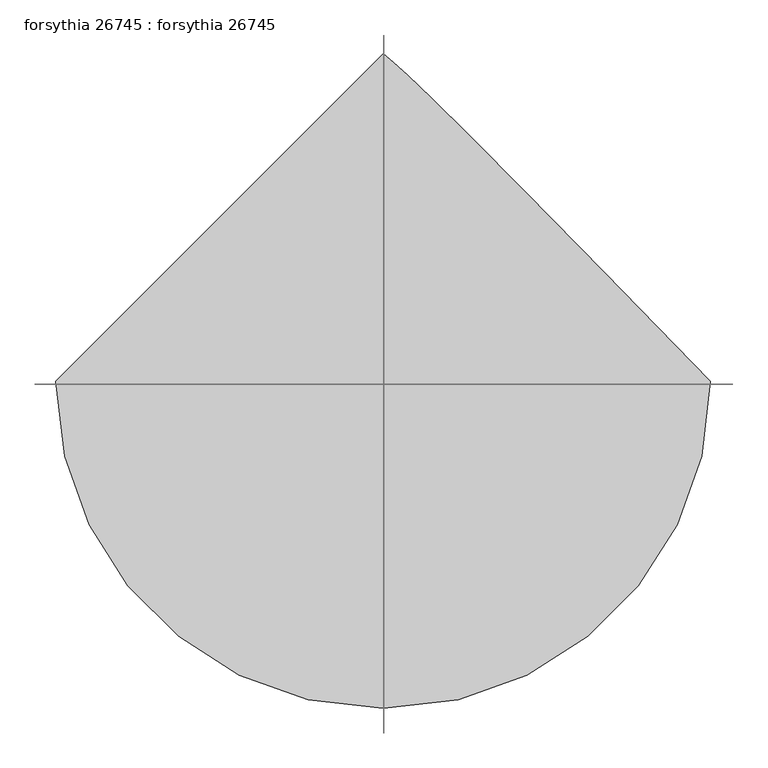
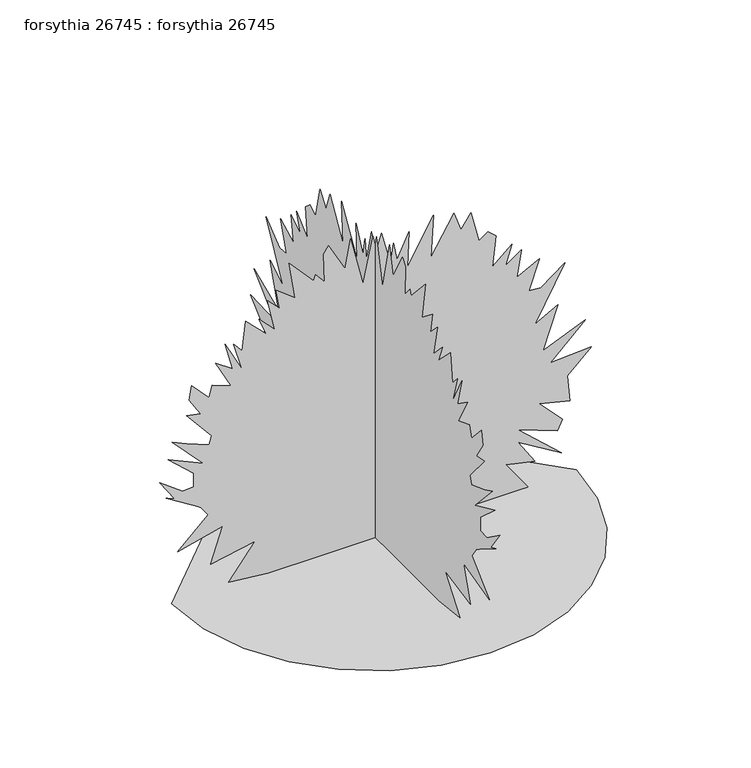
"""IFC4 building model written with IfcOpenShell, lengths in millimetres: proxy geometry, forsythia 26745 : forsythia 26745."""

from ifc_helpers import new_model, si_unit, origin, place, context, project, spatial, triangles, source, transform, mapped, element, save


def forsythia_26745_forsythia_26745_3ae10d36(model_context):
    return source(origin(), model_context, "Body", "Tessellation", [
        triangles([(-1519.5040535, 0.0, 0.0002833), (-1479.3336857, -348.1690825, 0.0002833), (-1364.9291862, -667.9078508, 0.0002833), (-1185.447191, -950.0545097, 0.0002833), (-950.0545097, -1185.447191, 0.0002833), (-667.9078508, -1364.9291862, 0.0002833), (-348.1690825, -1479.3336857, 0.0002833), (6.64e-05, -1519.5040535, 0.0002833), (348.1690825, -1479.3336857, 0.0002833), (667.9078508, -1364.9291862, 0.0002833), (950.0545097, -1185.447191, 0.0002833), (1185.447191, -950.0545097, 0.0002833), (1364.9291862, -667.9078508, 0.0002833), (1479.3336857, -348.1690825, 0.0002833), (1519.5040535, 0.0001328, 0.0002833), (1025.698439, 506.5233338, 0.0002833), (659.6172232, 879.4549673, 0.0002833), (399.9699903, 1141.05804, 0.0002833), (225.4722113, 1313.5981625, 0.0002833), (114.8360501, 1419.3438881, 0.0002833), (46.774248, 1480.5555588, 0.0002833), (-0.0001993, 1519.5040535, 0.0002833), (-792.3428427, -13.4822871, 0.037948), (-1099.2418425, -13.4822621, 31.9687972), (-901.0348274, -13.4822871, 287.7194292), (-1233.5117718, -13.4822871, 223.7813261), (-1143.9993576, -13.4822871, 492.3196223), (-1482.8669003, -13.4822871, 409.2003862), (-1252.691415, -13.482312, 620.1937574), (-1310.2352863, -13.482312, 703.3130299), (-1565.9861, -13.482312, 863.1557442), (-1502.0490143, -13.482312, 837.5804157), (-1617.1342861, -13.482312, 1003.8188152), (-1444.505143, -13.482312, 875.9446438), (-1361.3859432, -13.482312, 882.3378582), (-1361.3859432, -13.482312, 991.0299156), (-1553.1972004, -13.4823382, 1163.6615295), (-1291.0531723, -13.4823382, 1042.1805725), (-1521.2286575, -13.4823382, 1291.5383171), (-1412.5366001, -13.4823382, 1240.3875149), (-1246.2982006, -13.4823382, 1176.4505018), (-1227.1160866, -13.4823382, 1240.3875149), (-1412.5366001, -13.4823382, 1464.1673149), (-1310.2352863, -13.4823382, 1444.987817), (-1393.3544861, -13.4823631, 1579.2552029), (-1374.1723721, -13.4823631, 1687.9497311), (-1246.2982006, -13.4823631, 1547.28666), (-1220.7228722, -13.4823631, 1636.7990742), (-1080.0597284, -13.4823631, 1585.6482719), (-1195.147471, -13.4823631, 1803.0374737), (-1067.2732996, -13.4823631, 1713.5250595), (-1124.8171709, -13.4823881, 1930.9116451), (-996.9429995, -13.4823631, 1687.9497311), (-1060.8800852, -13.4823881, 1905.3363167), (-996.9429995, -13.4823631, 1835.0060165), (-971.367671, -13.4823881, 2058.7858166), (-817.9181711, -13.4823881, 1905.3363167), (-869.0663572, -13.4823881, 2039.6061733), (-753.9785419, -13.4823881, 1918.1252163), (-805.1292715, -13.4823881, 2161.0871304), (-715.6167847, -13.4823881, 2071.5747162), (-741.1921858, -13.4823881, 2225.0242161), (-600.5290421, -13.4823881, 2116.3296879), (-645.2865572, -13.4824142, 2404.0490444), (-459.8659347, -13.4823881, 2199.4488876), (-447.0795422, -13.4823881, 2244.2063301), (-379.2689283, -13.4823881, 2162.8804802), (-385.6646862, -13.4824142, 2386.6602802), (-347.290248, -13.4824142, 2438.4078484), (-223.176294, -13.4824142, 2213.9981449), (-182.9654127, -13.4823631, 2435.1743248), (-90.8322191, -13.4823631, 2047.6376598), (-12.3045871, -13.4824142, 2397.6559753), (13.2704245, -13.4823881, 2276.174873), (51.6330312, -13.4824142, 2397.6559753), (115.5706256, -13.4823881, 2135.5118019), (141.1454544, -13.4823881, 2288.9613018), (166.7205467, -13.4823881, 2148.2982307), (256.2334877, -13.4824142, 2340.1119587), (243.445551, -13.4823881, 2065.1815018), (441.6515305, -13.4824142, 2404.0490444), (422.4693801, -13.4823881, 2077.9679306), (595.1010303, -13.4824142, 2365.6874325), (646.2517599, -13.4823881, 2218.6310017), (722.9777452, -13.4824142, 2327.3230591), (780.5216166, -13.4823881, 2084.361145), (850.8519167, -13.4823881, 2129.1185875), (908.395788, -13.4823881, 2077.9679306), (882.8204596, -13.4823631, 1841.399231), (1029.876745, -13.4823881, 1969.2734024), (978.7260881, -13.4823631, 1815.8239025), (1100.2070452, -13.4823881, 1898.9431023), (1068.2385023, -13.4823631, 1694.3429455), (1234.4769745, -13.4823631, 1783.8553596), (1157.7509165, -13.4823631, 1553.6797291), (1247.2634033, -13.4823631, 1547.28666), (1426.2882317, -13.4823631, 1681.5565166), (1202.5084316, -13.4823382, 1272.3560577), (1375.1400455, -13.4823382, 1368.2616863), (1260.0523029, -13.4823382, 1042.1805725), (1579.7377316, -13.4823382, 1176.4505018), (1317.5961742, -13.482312, 927.0928299), (1624.495174, -13.482312, 946.2749439), (1445.4703457, -13.482312, 780.0364717), (1464.6524597, -13.4822871, 575.436315), (1234.4769745, -13.482312, 632.9801863), (1407.1085884, -13.4822871, 447.5621435), (1368.7443604, -13.4822871, 370.838629), (1074.6317167, -13.4822871, 479.5306864), (1400.7129032, -13.4822871, 185.418824), (1074.6317167, -13.4822871, 383.6250578), (1202.5084316, -13.4822871, 185.418824), (985.1193026, -13.4822871, 236.568736), (1151.4898161, -13.4822871, 0.0386752), (19.664159, -13.4822621, 0.0001234), (3.6800653, -809.5031324, 0.0378489), (3.68004, -1116.4046757, 31.9687972), (3.6800653, -918.1977333, 287.7194292), (3.6800653, -1250.6720615, 223.7813261), (3.6800653, -1161.1596474, 492.3196223), (3.6800653, -1500.0298061, 409.2003862), (3.6800653, -1269.8541756, 620.1937574), (3.6800653, -1327.3980469, 703.3130299), (3.6800908, -1583.1463898, 863.1557442), (3.6800908, -1519.209304, 837.5804157), (3.6800908, -1634.2970467, 1003.8188152), (3.6800908, -1461.6654327, 875.9446438), (3.6800908, -1378.5487038, 882.3378582), (3.6800908, -1378.5487038, 991.0299156), (3.6800908, -1570.3599609, 1163.6615295), (3.6800908, -1308.2159328, 1042.1805725), (3.6800908, -1538.3914181, 1291.5383171), (3.6800908, -1429.6968899, 1240.3875149), (3.6800908, -1263.4609612, 1176.4505018), (3.6800908, -1244.2788471, 1240.3875149), (3.6800908, -1429.6968899, 1464.1673149), (3.6800908, -1327.3980469, 1444.987817), (3.6800908, -1410.5172466, 1579.2552029), (3.6801161, -1391.3351326, 1687.9497311), (3.6800908, -1263.4609612, 1547.28666), (3.6800908, -1237.8856327, 1636.7990742), (3.6800908, -1097.2225616, 1585.6508881), (3.6801161, -1212.3103043, 1803.0374737), (3.6800908, -1084.4361328, 1713.5250595), (3.6801161, -1141.9800041, 1930.9116451), (3.6800908, -1014.1032892, 1687.9497311), (3.6801161, -1078.0403749, 1905.3363167), (3.6800908, -1014.1032892, 1835.0060165), (3.6801161, -988.5305042, 2058.7858166), (3.6800908, -835.0784609, 1905.3363167), (3.6801161, -886.2291904, 2039.6061733), (3.6800908, -771.1413752, 1918.1252163), (3.6801161, -822.2921047, 2161.0871304), (3.6801161, -732.7796179, 2071.5747162), (3.6801161, -758.355019, 2225.0242161), (3.6801161, -617.6918753, 2116.3296879), (3.6801161, -662.446847, 2404.0490444), (3.6801161, -477.0287679, 2199.4488876), (3.6801161, -464.2423754, 2244.2063301), (3.6801161, -396.4317616, 2162.8804802), (3.6801161, -402.824976, 2386.6602802), (3.6801161, -364.4530812, 2438.4078484), (3.6801161, -240.3386185, 2213.9981449), (3.6800653, -200.1277554, 2435.1743248), (3.6800653, -107.994798, 2047.640276), (3.6801161, -29.4668878, 2397.6559753), (3.6800908, -3.8919275, 2276.174873), (3.6801161, 34.4707044, 2397.6559753), (3.6800908, 98.408301, 2135.5118019), (3.6800908, 123.9831299, 2288.9613018), (3.6800908, 149.5579678, 2148.3008469), (3.6800908, 239.0706363, 2340.1119587), (3.6800908, 226.2832264, 2065.1815018), (3.6800908, 424.4886972, 2404.0490444), (3.6800908, 405.3090903, 2077.9679306), (3.6800908, 577.9381971, 2365.6874325), (3.6800908, 629.0889267, 2218.6310017), (3.6800908, 705.814912, 2327.3256752), (3.6800908, 763.3587833, 2084.361145), (3.6800908, 833.6890835, 2129.1185875), (3.6800908, 891.2329548, 2077.9679306), (3.6800653, 865.6576263, 1841.399231), (3.6800653, 1012.7139118, 1969.2734024), (3.6800653, 961.5632549, 1815.8239025), (3.6800653, 1083.044212, 1898.9431023), (3.6800653, 1051.0756691, 1694.3429455), (3.6800653, 1217.3141413, 1783.8553596), (3.6800653, 1140.5880833, 1553.6797291), (3.6800653, 1230.1004974, 1547.28666), (3.6800653, 1409.1253258, 1681.5565166), (3.6800653, 1185.3455984, 1272.3560577), (3.6800653, 1357.977285, 1368.2616863), (3.68004, 1242.8895424, 1042.1805725), (3.68004, 1562.5774418, 1176.4505018), (3.68004, 1300.4334137, 927.0928299), (3.68004, 1607.3324135, 946.2749439), (3.68004, 1428.3075851, 780.0364717), (3.68004, 1447.4896992, 575.436315), (3.68004, 1217.3141413, 632.9801863), (3.6800145, 1389.9458279, 447.5621435), (3.6800145, 1351.5840706, 370.838629), (3.68004, 1057.471427, 479.5306864), (3.6800145, 1383.5526134, 185.4185696), (3.68004, 1057.471427, 383.6250578), (3.6800145, 1185.3455984, 185.4185696), (3.6800145, 967.9590128, 236.568736), (3.68004, 1134.3269829, 0.038518), (3.68004, 2.5017556, 0.0)], [[21, 22, 1], [20, 21, 1], [19, 20, 1], [18, 19, 1], [17, 18, 1], [17, 1, 2], [17, 2, 3], [17, 3, 4], [16, 17, 4], [16, 4, 5], [16, 5, 6], [16, 6, 7], [16, 7, 8], [16, 8, 9], [16, 9, 10], [16, 10, 11], [16, 11, 12], [15, 16, 12], [14, 15, 12], [13, 14, 12], [30, 31, 32], [109, 110, 111], [51, 52, 53], [36, 37, 38], [32, 33, 34], [76, 77, 78], [100, 101, 102], [38, 39, 40], [78, 79, 80], [57, 58, 59], [70, 71, 72], [96, 97, 98], [72, 73, 74], [53, 54, 55], [80, 81, 82], [49, 50, 51], [27, 28, 29], [89, 90, 91], [74, 75, 76], [59, 60, 61], [63, 64, 65], [38, 40, 41], [102, 103, 104], [42, 43, 44], [98, 99, 100], [61, 62, 63], [93, 94, 95], [111, 112, 113], [91, 92, 93], [84, 85, 86], [82, 83, 84], [55, 56, 57], [45, 46, 47], [44, 45, 47], [113, 114, 115], [65, 66, 67], [23, 24, 25], [72, 74, 76], [25, 26, 27], [68, 69, 70], [67, 68, 70], [30, 32, 34], [30, 34, 35], [104, 105, 106], [49, 51, 53], [102, 104, 106], [95, 96, 98], [47, 48, 49], [107, 108, 109], [106, 107, 109], [82, 84, 86], [86, 87, 88], [86, 88, 89], [67, 70, 72], [115, 23, 25], [53, 55, 57], [82, 86, 89], [76, 78, 80], [63, 65, 67], [59, 61, 63], [42, 44, 47], [42, 47, 49], [35, 36, 38], [72, 76, 80], [111, 113, 115], [109, 111, 115], [100, 102, 106], [100, 106, 109], [100, 109, 115], [98, 100, 115], [98, 115, 25], [95, 98, 25], [93, 95, 25], [91, 93, 25], [89, 91, 25], [82, 89, 25], [80, 82, 25], [72, 80, 25], [72, 25, 27], [72, 27, 29], [67, 72, 29], [63, 67, 29], [59, 63, 29], [59, 29, 30], [59, 30, 35], [59, 35, 38], [59, 38, 41], [59, 41, 42], [59, 42, 49], [59, 49, 53], [59, 53, 57], [123, 124, 125], [202, 203, 204], [144, 145, 146], [129, 130, 131], [125, 126, 127], [169, 170, 171], [193, 194, 195], [131, 132, 133], [171, 172, 173], [150, 151, 152], [163, 164, 165], [189, 190, 191], [165, 166, 167], [146, 147, 148], [173, 174, 175], [142, 143, 144], [120, 121, 122], [182, 183, 184], [167, 168, 169], [152, 153, 154], [156, 157, 158], [131, 133, 134], [195, 196, 197], [135, 136, 137], [191, 192, 193], [154, 155, 156], [186, 187, 188], [204, 205, 206], [184, 185, 186], [177, 178, 179], [175, 176, 177], [148, 149, 150], [138, 139, 140], [137, 138, 140], [206, 207, 208], [158, 159, 160], [116, 117, 118], [165, 167, 169], [118, 119, 120], [161, 162, 163], [160, 161, 163], [123, 125, 127], [123, 127, 128], [197, 198, 199], [142, 144, 146], [195, 197, 199], [188, 189, 191], [140, 141, 142], [200, 201, 202], [199, 200, 202], [175, 177, 179], [179, 180, 181], [179, 181, 182], [160, 163, 165], [208, 116, 118], [146, 148, 150], [175, 179, 182], [169, 171, 173], [156, 158, 160], [152, 154, 156], [135, 137, 140], [135, 140, 142], [128, 129, 131], [165, 169, 173], [204, 206, 208], [202, 204, 208], [193, 195, 199], [193, 199, 202], [193, 202, 208], [191, 193, 208], [191, 208, 118], [188, 191, 118], [186, 188, 118], [184, 186, 118], [182, 184, 118], [175, 182, 118], [173, 175, 118], [165, 173, 118], [165, 118, 120], [165, 120, 122], [160, 165, 122], [156, 160, 122], [152, 156, 122], [152, 122, 123], [152, 123, 128], [152, 128, 131], [152, 131, 134], [152, 134, 135], [152, 135, 142], [152, 142, 146], [152, 146, 150]], closed=False),
    ])


if __name__ == "__main__":
    model = new_model("IFC4")
    model_context = context("Model", 3, world=origin())
    ifc_project = project(units=[si_unit("LENGTHUNIT", "METRE", prefix="MILLI")], contexts=[model_context])
    site = spatial("IfcSite", under=ifc_project)
    building = spatial("IfcBuilding", under=site)
    placement = place(None, origin())
    forsythia_26745_forsythia_26745_shape = forsythia_26745_forsythia_26745_3ae10d36(model_context)
    element("IfcBuildingElementProxy", 1, Name="forsythia 26745 : forsythia 26745", ObjectType="forsythia 26745 : forsythia 26745", at=placement, inside=building, context=model_context, shape_type="MappedRepresentation", body=[
        mapped(forsythia_26745_forsythia_26745_shape, transform((0.0, 0.0, 0.0), x_axis=(1.0, 0.0, 0.0), y_axis=(0.0, 1.0, 0.0), z_axis=(0.0, 0.0, 1.0))),
    ])
    save(model, "model.ifc")

# Revit data of these elements
# Type "forsythia 26745 : forsythia 26745"
#   built-in parameter 1005195 = "RPC-16-G2F6-877X-GLVN-N000-ST1L-LVER-AU"
#   Height = 0
